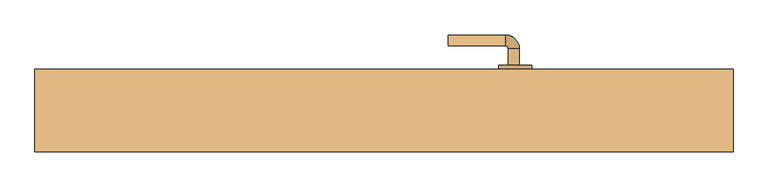
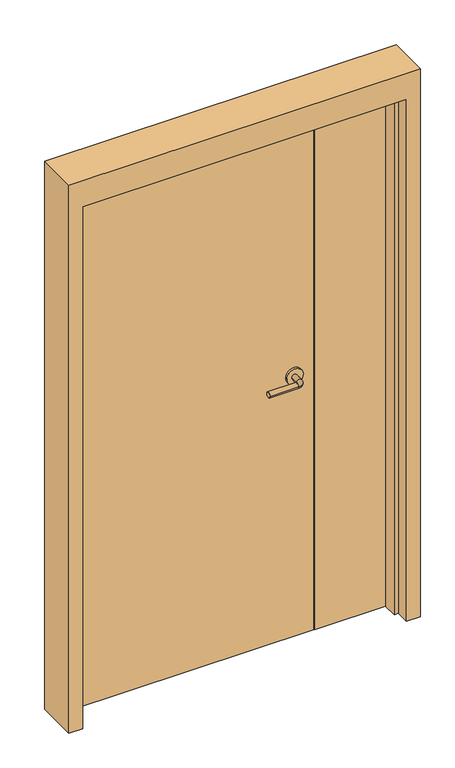
"""IFC4 building model written with IfcOpenShell, lengths in millimetres: door geometry, Дверь-Маятниковая-С полотнами разной ширины-Щитовая : 1275 x 2100 мм."""

from ifc_helpers import new_model, si_unit, point, frame, frame_2d, origin, origin_with_axes, place, context, project, spatial, polyline, circle_curve, ellipse_curve, trimmed, segment, composite_curve, outline, extrude, faceted_brep, source, transform, mapped, element, save
from ifc_brep_helpers import plane_surface, cylinder_surface, revolved_surface, advanced_brep


def door_0e9f5021(model_context):
    return source(origin(), model_context, "Body", "SolidModel", [
        advanced_brep(
        [(247.09375, 15.85, 1000.0), (227.09375, 15.85, 1000.0), (247.09375, -14.15, 1000.0), (227.09375, -14.15, 1000.0), (222.09375, -19.15, 1000.0), (222.09375, -39.15, 1000.0), (117.09375, -39.15, 1000.0), (117.09375, -19.15, 1000.0)],
        [
            (0, 1, circle_curve(frame((237.09375, 15.85, 1000.0), z_axis=(0.0, 1.0, 0.0), x_axis=(-1.0, 0.0, 0.0)), 10.0)),
            (1, 0, circle_curve(frame((237.09375, 15.85, 1000.0), z_axis=(0.0, 1.0, 0.0), x_axis=(-1.0, 0.0, 0.0)), 10.0)),
            (0, 2),
            (2, 3, circle_curve(frame((237.09375, -14.15, 1000.0), z_axis=(0.0, 1.0, 0.0), x_axis=(-1.0, 0.0, 0.0)), 10.0)),
            (3, 1),
            (3, 2, circle_curve(frame((237.09375, -14.15, 1000.0), z_axis=(0.0, 1.0, 0.0), x_axis=(-1.0, 0.0, 0.0)), 10.0)),
            (4, 3, circle_curve(frame((222.09375, -14.15, 1000.0), z_axis=(0.0, 0.0, 1.0), x_axis=(1.0, 0.0, 0.0)), 5.0)),
            (2, 5, circle_curve(frame((222.09375, -14.15, 1000.0), z_axis=(0.0, 0.0, -1.0), x_axis=(1.0, 0.0, 0.0)), 25.0)),
            (5, 4, circle_curve(frame((222.09375, -29.15, 1000.0), z_axis=(1.0, 0.0, 0.0), x_axis=(0.0, 1.0, 0.0)), 10.0)),
            (4, 5, circle_curve(frame((222.09375, -29.15, 1000.0), z_axis=(1.0, 0.0, 0.0), x_axis=(0.0, 1.0, 0.0)), 10.0)),
            (6, 7, circle_curve(frame((117.09375, -29.15, 1000.0), z_axis=(-1.0, 0.0, 0.0), x_axis=(0.0, 1.0, 0.0)), 10.0)),
            (7, 6, circle_curve(frame((117.09375, -29.15, 1000.0), z_axis=(-1.0, 0.0, 0.0), x_axis=(0.0, 1.0, 0.0)), 10.0)),
            (5, 6),
            (7, 4),
        ],
        [
            plane_surface(frame((237.09375, 15.85, 1000.0), z_axis=(0.0, 1.0, 0.0), x_axis=(0.0, 0.0, 1.0))),
            cylinder_surface(frame((237.09375, 15.85, 1000.0), z_axis=(0.0, 1.0, 0.0), x_axis=(-1.0, 0.0, 0.0)), 10.0),
            revolved_surface(trimmed(ellipse_curve(frame((237.09375, -14.15, 1000.0), z_axis=(0.0, 1.0, 0.0), x_axis=(-1.0, 0.0, 0.0)), 10.0, 10.0), [point((247.09375, -14.15, 1000.0))], [point((227.09375, -14.15, 1000.0))], True, "CARTESIAN"), (222.09375, -14.15, 1000.0), (0.0, 0.0, -1.0)),
            revolved_surface(trimmed(ellipse_curve(frame((237.09375, -14.15, 1000.0), z_axis=(0.0, 1.0, 0.0), x_axis=(-1.0, 0.0, 0.0)), 10.0, 10.0), [point((227.09375, -14.15, 1000.0))], [point((247.09375, -14.15, 1000.0))], True, "CARTESIAN"), (222.09375, -14.15, 1000.0), (0.0, 0.0, -1.0)),
            plane_surface(frame((117.09375, -29.15, 1000.0), z_axis=(-1.0, 0.0, 0.0), x_axis=(0.0, 0.0, 1.0))),
            cylinder_surface(frame((222.09375, -29.15, 1000.0), z_axis=(1.0, 0.0, 0.0), x_axis=(0.0, 1.0, 0.0)), 10.0),
        ],
        [
            (0, [[1, 2]]),
            (1, [[-1, 3, 4, 5]]),
            (1, [[-2, -5, 6, -3]]),
            (2, [[7, -4, 8, 9]]),
            (3, [[-8, -6, -7, 10]]),
            (4, [[11, 12]]),
            (5, [[-9, 13, -12, 14]]),
            (5, [[-10, -14, -11, -13]]),
        ],
    ),
        extrude(outline(composite_curve([segment(trimmed(circle_curve(frame_2d((1000.0, 239.59375)), 30.0), [point((1000.0, 269.59375))], [point((1000.0, 209.59375))], False, "CARTESIAN"), True, "CONTINUOUS"), segment(trimmed(circle_curve(frame_2d((1000.0, 239.59375)), 30.0), [point((1000.0, 209.59375))], [point((1000.0, 269.59375))], False, "CARTESIAN"), True, "CONTINUOUS")], self_intersect=False)), frame((0.0, 15.85, 0.0), z_axis=(0.0, 1.0, 0.0), x_axis=(0.0, 0.0, 1.0)), (0.0, 0.0, 1.0), 8.0),
        advanced_brep(
        [(247.09375, 76.85, 1000.0), (227.09375, 76.85, 1000.0), (227.09375, 106.85, 1000.0), (247.09375, 106.85, 1000.0), (222.09375, 111.85, 1000.0), (222.09375, 131.85, 1000.0), (117.09375, 131.85, 1000.0), (117.09375, 111.85, 1000.0)],
        [
            (0, 1, circle_curve(frame((237.09375, 76.85, 1000.0), z_axis=(0.0, -1.0, 0.0), x_axis=(-1.0, 0.0, 0.0)), 10.0)),
            (1, 0, circle_curve(frame((237.09375, 76.85, 1000.0), z_axis=(0.0, -1.0, 0.0), x_axis=(-1.0, 0.0, 0.0)), 10.0)),
            (1, 2),
            (2, 3, circle_curve(frame((237.09375, 106.85, 1000.0), z_axis=(0.0, -1.0, 0.0), x_axis=(-1.0, 0.0, 0.0)), 10.0)),
            (3, 0),
            (3, 2, circle_curve(frame((237.09375, 106.85, 1000.0), z_axis=(0.0, -1.0, 0.0), x_axis=(-1.0, 0.0, 0.0)), 10.0)),
            (4, 5, circle_curve(frame((222.09375, 121.85, 1000.0), z_axis=(1.0, 0.0, 0.0), x_axis=(0.0, -1.0, 0.0)), 10.0)),
            (5, 3, circle_curve(frame((222.09375, 106.85, 1000.0), z_axis=(0.0, 0.0, -1.0), x_axis=(1.0, 0.0, 0.0)), 25.0)),
            (2, 4, circle_curve(frame((222.09375, 106.85, 1000.0), z_axis=(0.0, 0.0, 1.0), x_axis=(1.0, 0.0, 0.0)), 5.0)),
            (5, 4, circle_curve(frame((222.09375, 121.85, 1000.0), z_axis=(1.0, 0.0, 0.0), x_axis=(0.0, -1.0, 0.0)), 10.0)),
            (6, 7, circle_curve(frame((117.09375, 121.85, 1000.0), z_axis=(-1.0, 0.0, 0.0), x_axis=(0.0, -1.0, 0.0)), 10.0)),
            (7, 6, circle_curve(frame((117.09375, 121.85, 1000.0), z_axis=(-1.0, 0.0, 0.0), x_axis=(0.0, -1.0, 0.0)), 10.0)),
            (4, 7),
            (6, 5),
        ],
        [
            plane_surface(frame((237.09375, 76.85, 1000.0), z_axis=(0.0, -1.0, 0.0), x_axis=(0.0, 0.0, 1.0))),
            cylinder_surface(frame((237.09375, 76.85, 1000.0), z_axis=(0.0, -1.0, 0.0), x_axis=(-1.0, 0.0, 0.0)), 10.0),
            revolved_surface(trimmed(ellipse_curve(frame((237.09375, 106.85, 1000.0), z_axis=(0.0, 1.0, 0.0), x_axis=(-1.0, 0.0, 0.0)), 10.0, 10.0), [point((247.09375, 106.85, 1000.0))], [point((227.09375, 106.85, 1000.0))], True, "CARTESIAN"), (222.09375, 106.85, 1000.0), (0.0, 0.0, -1.0)),
            revolved_surface(trimmed(ellipse_curve(frame((237.09375, 106.85, 1000.0), z_axis=(0.0, 1.0, 0.0), x_axis=(-1.0, 0.0, 0.0)), 10.0, 10.0), [point((227.09375, 106.85, 1000.0))], [point((247.09375, 106.85, 1000.0))], True, "CARTESIAN"), (222.09375, 106.85, 1000.0), (0.0, 0.0, -1.0)),
            plane_surface(frame((117.09375, 121.85, 1000.0), z_axis=(-1.0, 0.0, 0.0), x_axis=(0.0, 0.0, 1.0))),
            cylinder_surface(frame((222.09375, 121.85, 1000.0), z_axis=(1.0, 0.0, 0.0), x_axis=(0.0, -1.0, 0.0)), 10.0),
        ],
        [
            (0, [[1, 2]]),
            (1, [[3, 4, 5, -2]]),
            (1, [[-5, 6, -3, -1]]),
            (2, [[7, 8, -4, 9]]),
            (3, [[10, -9, -6, -8]]),
            (4, [[11, 12]]),
            (5, [[13, -11, 14, -7]]),
            (5, [[-14, -12, -13, -10]]),
        ],
    ),
        extrude(outline(composite_curve([segment(trimmed(circle_curve(frame_2d((1000.0, 239.59375)), 30.0), [point((1000.0, 269.59375))], [point((1000.0, 209.59375))], False, "CARTESIAN"), True, "CONTINUOUS"), segment(trimmed(circle_curve(frame_2d((1000.0, 239.59375)), 30.0), [point((1000.0, 209.59375))], [point((1000.0, 269.59375))], False, "CARTESIAN"), True, "CONTINUOUS")], self_intersect=False)), frame((0.0, 68.85, 0.0), z_axis=(0.0, 1.0, 0.0), x_axis=(0.0, 0.0, 1.0)), (0.0, 0.0, 1.0), 8.0),
        extrude(outline(polyline([(587.5, 23.85), (314.1, 23.85), (314.1, 68.85), (587.5, 68.85), (587.5, 23.85)])), origin_with_axes(), (0.0, 0.0, 1.0), 2000.0),
        faceted_brep([(587.5, 19.0875, 0.0), (587.5, 68.85, 0.0), (637.5, 68.85, 0.0), (637.5, -81.15, 0.0), (587.5, -81.15, 0.0), (587.5, -31.9375, 0.0), (571.625, -31.9375, 0.0), (571.625, 19.0875, 0.0), (587.5, 19.0875, 2000.0), (587.5, 68.85, 2000.0), (-587.5, 68.85, 2000.0), (-587.5, 68.85, 0.0), (-637.5, 68.85, 0.0), (-637.5, 68.85, 2100.0), (637.5, 68.85, 2100.0), (637.5, -81.15, 2100.0), (-637.5, -81.15, 2100.0), (-637.5, -81.15, 0.0), (-587.5, -81.15, 0.0), (-587.5, -81.15, 2000.0), (587.5, -81.15, 2000.0), (587.5, -31.9375, 2000.0), (-587.5, -31.9375, 2000.0), (-587.5, -31.9375, 0.0), (-571.625, -31.9375, 0.0), (-571.625, -31.9375, 1984.125), (571.625, -31.9375, 1984.125), (571.625, 19.0875, 1984.125), (-571.625, 19.0875, 1984.125), (-571.625, 19.0875, 0.0), (-587.5, 19.0875, 0.0), (-587.5, 19.0875, 2000.0)], [[[0, 1, 2, 3, 4, 5, 6, 7]], [[1, 0, 8, 9]], [[2, 1, 9, 10, 11, 12, 13, 14]], [[3, 2, 14, 15]], [[4, 3, 15, 16, 17, 18, 19, 20]], [[5, 4, 20, 21]], [[6, 5, 21, 22, 23, 24, 25, 26]], [[7, 6, 26, 27]], [[0, 7, 27, 28, 29, 30, 31, 8]], [[9, 8, 31, 10]], [[20, 19, 22, 21]], [[26, 25, 28, 27]], [[12, 11, 30, 29, 24, 23, 18, 17]], [[11, 10, 31, 30]], [[13, 12, 17, 16]], [[19, 18, 23, 22]], [[25, 24, 29, 28]], [[15, 14, 13, 16]]]),
        extrude(outline(polyline([(310.9, 23.85), (-587.5, 23.85), (-587.5, 68.85), (310.9, 68.85), (310.9, 23.85)])), origin_with_axes(), (0.0, 0.0, 1.0), 2000.0),
    ])


if __name__ == "__main__":
    model = new_model("IFC4")
    model_context = context("Model", 3, world=origin())
    ifc_project = project(units=[si_unit("LENGTHUNIT", "METRE", prefix="MILLI")], contexts=[model_context])
    site = spatial("IfcSite", under=ifc_project)
    building = spatial("IfcBuilding", under=site)
    placement = place(None, origin())
    door_shape = door_0e9f5021(model_context)
    element("IfcDoor", 1, ObjectType="Дверь-Маятниковая-С полотнами разной ширины-Щитовая : 1275 x 2100 мм", at=placement, inside=building, context=model_context, shape_type="MappedRepresentation", body=[
        mapped(door_shape, transform((0.0, 0.0, 0.0), x_axis=(1.0, 0.0, 0.0), y_axis=(0.0, 1.0, 0.0), z_axis=(0.0, 0.0, 1.0))),
    ])
    save(model, "model.ifc")

# Revit data of these elements
# Type "Дверь-Маятниковая-С полотнами разной ширины-Щитовая : 1275 x 2100 мм"
#   Type Mark = "154"
#   Assembly Code = "C1020300"
#   Analytic Construction = "Деревянный"
#   Ширина большой панели = 900 mm
#   W = 275 mm
#   Thickness = 45 mm
#   Thermal Resistance (R) = 0.455703 (m²·K)/W
#   Угол поворота [instance default] = 90°
#   Высота планки = 1000 mm
#   Rough Width [instance default] = 1275 mm
#   Rough Height [instance default] = 2100 mm
#   Высота проема в кирпичном каркасе [instance default] = 100 mm
#   Ширина проема в кирпичном каркасе [instance default] = 100 mm
#   Расчет вставки [instance default] = 105 mm
#   Кирпичная вставка [instance default] = 25 mm
#   Height = 2000 mm
#   Width = 1175 mm
#   Heat Transfer Coefficient (U) = 2.19465 W/(m²·K)
#   Глубина кирпичного каркаса = 150 mm
#   Кирпичный каркас [instance default] = yes
#   Каркас стены сухой кладки [instance default] = no
#   Материал панели = Древесина - Береза
#   Материал каркаса = Металл - Окрашенный - Серый 2
#   Материал дверной ручки = Алюминий
#   Visual Light Transmittance = 0
#   Solar Heat Gain Coefficient = 0
#   Wall Closure = (empty or 0)
#   Function = (empty or 0)
# Element 1 (IfcDoor, "Дверь-Маятниковая-С полотнами разной ширины-Щитовая : 1275 x 2100 мм")
#   Расчет вставки = 80 mm
#   Кирпичная вставка = 0 mm
#   Materials on its faces: "Алюминий", "Металл - Окрашенный - Серый 2", "Древесина - Береза"
# Materials
#   "Древесина - Береза": class "Древесина", colour RGB 166 116 52, transparency 0, Cost = 0
#   "Металл - Окрашенный - Серый 2": class "Краска", colour RGB 104 104 104, transparency 0, Cost = 0
#   "Алюминий": class "Металл", colour RGB 247 247 247, transparency 0
